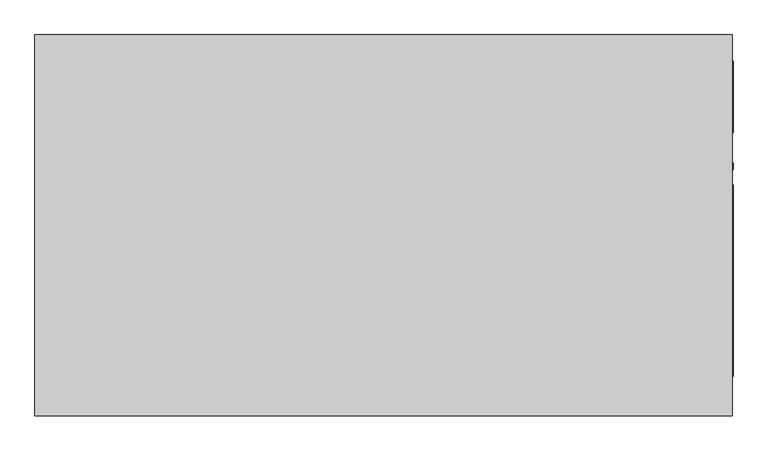
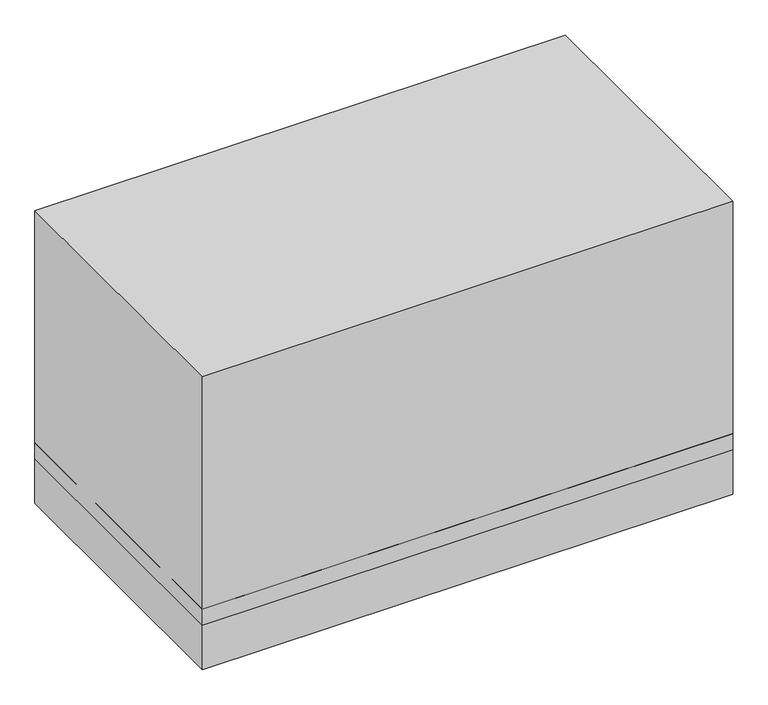
"""IFC4 building model written with IfcOpenShell, lengths in millimetres: proxy geometry, Carrier_48TC_Standard_Efficiency_Gas_Heat_Electric_Cooling_Packaged_Rooftop_Unit_3_to_15_nominal_tons : 15 ton 48TC**16."""

from ifc_helpers import new_model, si_unit, point, frame, frame_2d, origin, origin_with_axes, place, context, project, spatial, polyline, circle_curve, trimmed, segment, composite_curve, outline, extrude, source, transform, mapped, element, save
from ifc_brep_helpers import plane_surface, revolved_surface, advanced_brep


def mechanical_equipment_2a90b6eb(model_context):
    return source(origin(), model_context, "Body", "SolidModel", [
        extrude(outline(composite_curve([segment(trimmed(circle_curve(frame_2d((249.2375, 434.975)), 13.2953125), [point((235.9421875, 434.975))], [point((262.5328125, 434.975))], False, "CARTESIAN"), True, "CONTINUOUS"), segment(trimmed(circle_curve(frame_2d((249.2375, 434.975)), 13.2953125), [point((262.5328125, 434.975))], [point((235.9421875, 434.975))], False, "CARTESIAN"), True, "CONTINUOUS")], self_intersect=False)), frame((1471.6125, 0.0, 0.0), z_axis=(1.0, 0.0, 0.0), x_axis=(0.0, 1.0, 0.0)), (0.0, 0.0, 1.0), 3.175),
        advanced_brep(
        [(1471.6125, 804.8625, 1717.675), (-1471.6125, 804.8625, 1717.675), (-1471.6125, -804.8625, 1717.675), (1471.6125, -804.8625, 1717.675), (1471.6125, 804.8625, 260.35), (1471.6125, -804.8625, 260.35), (-1471.6125, -804.8625, 260.35), (-1471.6125, 804.8625, 260.35), (1312.8625, -681.0375, 260.35), (1312.8625, 0.0, 260.35), (633.4125, 0.0, 260.35), (633.4125, -681.0375, 260.35), (1312.8625, 642.9375, 260.35), (122.2375, 642.9375, 260.35), (122.2375, 322.2625, 260.35), (1312.8625, 322.2625, 260.35), (430.8078125, -144.4625, 260.35), (404.2171875, -144.4625, 260.35), (-336.55, -423.8625, 260.35), (-358.775, -423.8625, 260.35), (-315.9125, -344.4875, 260.35), (-379.4125, -344.4875, 260.35), (-325.4375, -233.3625, 260.35), (-369.8875, -233.3625, 260.35), (1312.8625, -681.0375, 381.0), (633.4125, -681.0375, 381.0), (633.4125, 0.0, 381.0), (1312.8625, 0.0, 381.0), (1312.8625, 642.9375, 381.0), (1312.8625, 322.2625, 381.0), (122.2375, 322.2625, 381.0), (122.2375, 642.9375, 381.0), (430.8078125, -144.4625, 415.925), (404.2171875, -144.4625, 415.925), (-336.55, -423.8625, 415.925), (-358.775, -423.8625, 415.925), (-315.9125, -344.4875, 415.925), (-379.4125, -344.4875, 415.925), (-325.4375, -233.3625, 415.925), (-369.8875, -233.3625, 415.925)],
        [
            (0, 1),
            (1, 2),
            (2, 3),
            (3, 0),
            (4, 5),
            (5, 6),
            (6, 7),
            (7, 4),
            (8, 9),
            (9, 10),
            (10, 11),
            (11, 8),
            (12, 13),
            (13, 14),
            (14, 15),
            (15, 12),
            (16, 17, circle_curve(frame((417.5125, -144.4625, 260.35), z_axis=(0.0, 0.0, 1.0), x_axis=(-1.0, 0.0, 0.0)), 13.2953125)),
            (17, 16, circle_curve(frame((417.5125, -144.4625, 260.35), z_axis=(0.0, 0.0, 1.0), x_axis=(-1.0, 0.0, 0.0)), 13.2953125)),
            (18, 19, circle_curve(frame((-347.6625, -423.8625, 260.35), z_axis=(0.0, 0.0, 1.0), x_axis=(-1.0, 0.0, 0.0)), 11.1125)),
            (19, 18, circle_curve(frame((-347.6625, -423.8625, 260.35), z_axis=(0.0, 0.0, 1.0), x_axis=(-1.0, 0.0, 0.0)), 11.1125)),
            (20, 21, circle_curve(frame((-347.6625, -344.4875, 260.35), z_axis=(0.0, 0.0, 1.0), x_axis=(-1.0, 0.0, 0.0)), 31.75)),
            (21, 20, circle_curve(frame((-347.6625, -344.4875, 260.35), z_axis=(0.0, 0.0, 1.0), x_axis=(-1.0, 0.0, 0.0)), 31.75)),
            (22, 23, circle_curve(frame((-347.6625, -233.3625, 260.35), z_axis=(0.0, 0.0, 1.0), x_axis=(-1.0, 0.0, 0.0)), 22.225)),
            (23, 22, circle_curve(frame((-347.6625, -233.3625, 260.35), z_axis=(0.0, 0.0, 1.0), x_axis=(-1.0, 0.0, 0.0)), 22.225)),
            (0, 4),
            (7, 1),
            (6, 2),
            (5, 3),
            (24, 25),
            (25, 26),
            (26, 27),
            (27, 24),
            (27, 9),
            (8, 24),
            (26, 10),
            (25, 11),
            (28, 29),
            (29, 30),
            (30, 31),
            (31, 28),
            (31, 13),
            (12, 28),
            (30, 14),
            (29, 15),
            (32, 33, circle_curve(frame((417.5125, -144.4625, 415.925), z_axis=(0.0, 0.0, -1.0), x_axis=(-1.0, 0.0, 0.0)), 13.2953125)),
            (33, 32, circle_curve(frame((417.5125, -144.4625, 415.925), z_axis=(0.0, 0.0, -1.0), x_axis=(-1.0, 0.0, 0.0)), 13.2953125)),
            (33, 17),
            (16, 32),
            (34, 35, circle_curve(frame((-347.6625, -423.8625, 415.925), z_axis=(0.0, 0.0, -1.0), x_axis=(-1.0, 0.0, 0.0)), 11.1125)),
            (35, 34, circle_curve(frame((-347.6625, -423.8625, 415.925), z_axis=(0.0, 0.0, -1.0), x_axis=(-1.0, 0.0, 0.0)), 11.1125)),
            (35, 19),
            (18, 34),
            (36, 37, circle_curve(frame((-347.6625, -344.4875, 415.925), z_axis=(0.0, 0.0, -1.0), x_axis=(-1.0, 0.0, 0.0)), 31.75)),
            (37, 36, circle_curve(frame((-347.6625, -344.4875, 415.925), z_axis=(0.0, 0.0, -1.0), x_axis=(-1.0, 0.0, 0.0)), 31.75)),
            (37, 21),
            (20, 36),
            (38, 39, circle_curve(frame((-347.6625, -233.3625, 415.925), z_axis=(0.0, 0.0, -1.0), x_axis=(-1.0, 0.0, 0.0)), 22.225)),
            (39, 38, circle_curve(frame((-347.6625, -233.3625, 415.925), z_axis=(0.0, 0.0, -1.0), x_axis=(-1.0, 0.0, 0.0)), 22.225)),
            (39, 23),
            (22, 38),
        ],
        [
            plane_surface(frame((-1471.6125, 804.8625, 1717.675), z_axis=(0.0, 0.0, 1.0), x_axis=(-1.0, 0.0, 0.0))),
            plane_surface(frame((-1471.6125, 804.8625, 260.35), z_axis=(0.0, 0.0, -1.0), x_axis=(1.0, 0.0, 0.0))),
            plane_surface(frame((1471.6125, 804.8625, 1717.675), z_axis=(0.0, 1.0, 0.0), x_axis=(0.0, 0.0, -1.0))),
            plane_surface(frame((-1471.6125, 804.8625, 1717.675), z_axis=(-1.0, 0.0, 0.0), x_axis=(0.0, 0.0, -1.0))),
            plane_surface(frame((-1471.6125, -804.8625, 1717.675), z_axis=(0.0, -1.0, 0.0), x_axis=(0.0, 0.0, -1.0))),
            plane_surface(frame((1471.6125, -804.8625, 1717.675), z_axis=(1.0, 0.0, 0.0), x_axis=(0.0, 0.0, -1.0))),
            plane_surface(frame((1312.8625, -681.0375, 381.0), z_axis=(0.0, 0.0, -1.0), x_axis=(0.0, 1.0, 0.0))),
            plane_surface(frame((1312.8625, -681.0375, 381.0), z_axis=(-1.0, 0.0, 0.0), x_axis=(0.0, 0.0, -1.0))),
            plane_surface(frame((1312.8625, 0.0, 381.0), z_axis=(0.0, -1.0, 0.0), x_axis=(0.0, 0.0, -1.0))),
            plane_surface(frame((633.4125, 0.0, 381.0), z_axis=(1.0, 0.0, 0.0), x_axis=(0.0, 0.0, -1.0))),
            plane_surface(frame((633.4125, -681.0375, 381.0), z_axis=(0.0, 1.0, 0.0), x_axis=(0.0, 0.0, -1.0))),
            plane_surface(frame((122.2375, 642.9375, 381.0), z_axis=(0.0, 0.0, -1.0), x_axis=(-1.0, 0.0, 0.0))),
            plane_surface(frame((1312.8625, 642.9375, 381.0), z_axis=(0.0, -1.0, 0.0), x_axis=(0.0, 0.0, -1.0))),
            plane_surface(frame((122.2375, 642.9375, 381.0), z_axis=(1.0, 0.0, 0.0), x_axis=(0.0, 0.0, -1.0))),
            plane_surface(frame((122.2375, 322.2625, 381.0), z_axis=(0.0, 1.0, 0.0), x_axis=(0.0, 0.0, -1.0))),
            plane_surface(frame((1312.8625, 322.2625, 381.0), z_axis=(-1.0, 0.0, 0.0), x_axis=(0.0, 0.0, -1.0))),
            plane_surface(frame((404.2171875, -144.4625, 415.925), z_axis=(0.0, 0.0, -1.0), x_axis=(0.0, -1.0, 0.0))),
            revolved_surface(polyline([(404.21718749999997, -144.4625, 415.925), (404.21718749999997, -144.4625, 260.35)]), (417.5125, -144.4625, 0.0), (0.0, 0.0, 1.0)),
            plane_surface(frame((-358.775, -423.8625, 415.925), z_axis=(0.0, 0.0, -1.0), x_axis=(0.0, -1.0, 0.0))),
            revolved_surface(polyline([(-358.77500000000003, -423.8625, 415.925), (-358.77500000000003, -423.8625, 260.35)]), (-347.6625, -423.8625, 0.0), (0.0, 0.0, 1.0)),
            plane_surface(frame((-379.4125, -344.4875, 415.925), z_axis=(0.0, 0.0, -1.0), x_axis=(0.0, -1.0, 0.0))),
            revolved_surface(polyline([(-379.4125, -344.4875, 415.925), (-379.4125, -344.4875, 260.35)]), (-347.6625, -344.4875, 0.0), (0.0, 0.0, 1.0)),
            plane_surface(frame((-369.8875, -233.3625, 415.925), z_axis=(0.0, 0.0, -1.0), x_axis=(0.0, -1.0, 0.0))),
            revolved_surface(polyline([(-369.88750000000005, -233.3625, 415.925), (-369.88750000000005, -233.3625, 260.35)]), (-347.6625, -233.3625, 0.0), (0.0, 0.0, 1.0)),
        ],
        [
            (0, [[1, 2, 3, 4]]),
            (1, [[5, 6, 7, 8], [9, 10, 11, 12], [13, 14, 15, 16], [17, 18], [19, 20], [21, 22], [23, 24]]),
            (2, [[-1, 25, -8, 26]]),
            (3, [[-2, -26, -7, 27]]),
            (4, [[-3, -27, -6, 28]]),
            (5, [[-4, -28, -5, -25]]),
            (6, [[29, 30, 31, 32]]),
            (7, [[-32, 33, -9, 34]]),
            (8, [[-31, 35, -10, -33]]),
            (9, [[-30, 36, -11, -35]]),
            (10, [[-29, -34, -12, -36]]),
            (11, [[37, 38, 39, 40]]),
            (12, [[-40, 41, -13, 42]]),
            (13, [[-39, 43, -14, -41]]),
            (14, [[-38, 44, -15, -43]]),
            (15, [[-37, -42, -16, -44]]),
            (16, [[45, 46]]),
            (17, [[-46, 47, -17, 48]]),
            (17, [[-45, -48, -18, -47]]),
            (18, [[49, 50]]),
            (19, [[-50, 51, -19, 52]]),
            (19, [[-49, -52, -20, -51]]),
            (20, [[53, 54]]),
            (21, [[-54, 55, -21, 56]]),
            (21, [[-53, -56, -22, -55]]),
            (22, [[57, 58]]),
            (23, [[-58, 59, -23, 60]]),
            (23, [[-57, -60, -24, -59]]),
        ],
    ),
        extrude(outline(polyline([(1471.6125, 804.8625), (1471.6125, -804.8625), (-1471.6125, -804.8625), (-1471.6125, 804.8625), (1471.6125, 804.8625)]), holes=[polyline([(1312.8625, 642.9375), (122.2375, 642.9375), (122.2375, 322.2625), (1312.8625, 322.2625), (1312.8625, 642.9375)]), polyline([(1312.8625, -681.0375), (1312.8625, 0.0), (633.4125, 0.0), (633.4125, -681.0375), (1312.8625, -681.0375)]), composite_curve([segment(trimmed(circle_curve(frame_2d((417.5125, -144.4625)), 13.2953125), [point((430.8078125, -144.4625))], [point((404.2171875, -144.4625))], True, "CARTESIAN"), True, "CONTINUOUS"), segment(trimmed(circle_curve(frame_2d((417.5125, -144.4625)), 13.2953125), [point((404.2171875, -144.4625))], [point((430.8078125, -144.4625))], True, "CARTESIAN"), True, "CONTINUOUS")], self_intersect=False), composite_curve([segment(trimmed(circle_curve(frame_2d((-347.6625, -423.8625)), 11.1125), [point((-336.55, -423.8625))], [point((-358.775, -423.8625))], True, "CARTESIAN"), True, "CONTINUOUS"), segment(trimmed(circle_curve(frame_2d((-347.6625, -423.8625)), 11.1125), [point((-358.775, -423.8625))], [point((-336.55, -423.8625))], True, "CARTESIAN"), True, "CONTINUOUS")], self_intersect=False), composite_curve([segment(trimmed(circle_curve(frame_2d((-347.6625, -344.4875)), 31.75), [point((-315.9125, -344.4875))], [point((-379.4125, -344.4875))], True, "CARTESIAN"), True, "CONTINUOUS"), segment(trimmed(circle_curve(frame_2d((-347.6625, -344.4875)), 31.75), [point((-379.4125, -344.4875))], [point((-315.9125, -344.4875))], True, "CARTESIAN"), True, "CONTINUOUS")], self_intersect=False), composite_curve([segment(trimmed(circle_curve(frame_2d((-347.6625, -233.3625)), 22.225), [point((-325.4375, -233.3625))], [point((-369.8875, -233.3625))], True, "CARTESIAN"), True, "CONTINUOUS"), segment(trimmed(circle_curve(frame_2d((-347.6625, -233.3625)), 22.225), [point((-369.8875, -233.3625))], [point((-325.4375, -233.3625))], True, "CARTESIAN"), True, "CONTINUOUS")], self_intersect=False)]), origin_with_axes(), (0.0, 0.0, 1.0), 355.6),
        extrude(outline(polyline([(1474.7875, 693.7375), (1474.7875, 392.1125), (1471.6125, 392.1125), (1471.6125, 693.7375), (1474.7875, 693.7375)])), frame((0.0, 0.0, 415.925), z_axis=(0.0, 0.0, 1.0), x_axis=(1.0, 0.0, 0.0)), (0.0, 0.0, 1.0), 1171.575),
        extrude(outline(polyline([(1474.7875, 169.8625), (1474.7875, -636.5875), (1471.6125, -636.5875), (1471.6125, 169.8625), (1474.7875, 169.8625)])), frame((0.0, 0.0, 415.925), z_axis=(0.0, 0.0, 1.0), x_axis=(1.0, 0.0, 0.0)), (0.0, 0.0, 1.0), 371.475),
    ])


if __name__ == "__main__":
    model = new_model("IFC4")
    model_context = context("Model", 3, world=origin())
    ifc_project = project(units=[si_unit("LENGTHUNIT", "METRE", prefix="MILLI")], contexts=[model_context])
    site = spatial("IfcSite", under=ifc_project)
    building = spatial("IfcBuilding", under=site)
    placement = place(None, origin())
    mechanical_equipment_shape = mechanical_equipment_2a90b6eb(model_context)
    element("IfcBuildingElementProxy", 1, Name="Carrier_48TC_Standard_Efficiency_Gas_Heat_Electric_Cooling_Packaged_Rooftop_Unit_3_to_15_nominal_tons : 15 ton 48TC**16", ObjectType="Carrier_48TC_Standard_Efficiency_Gas_Heat_Electric_Cooling_Packaged_Rooftop_Unit_3_to_15_nominal_tons : 15 ton 48TC**16", at=placement, inside=building, context=model_context, shape_type="MappedRepresentation", body=[
        mapped(mechanical_equipment_shape, transform((0.0, 0.0, 0.0), x_axis=(1.0, 0.0, 0.0), y_axis=(0.0, 1.0, 0.0), z_axis=(0.0, 0.0, 1.0))),
    ])
    save(model, "model.ifc")

# Revit data of these elements
# Type "Carrier_48TC_Standard_Efficiency_Gas_Heat_Electric_Cooling_Packaged_Rooftop_Unit_3_to_15_nominal_tons : 15 ton 48TC**16"
#   URL = "www.Carrier.com"
#   Model = "48TC"
#   Manufacturer = "Carrier"
#   Disclaimer = "Manufacturer reserves the right to change, at any time, specifications and designs without notice and without obligation.  Please verify critical parameters with local Carrier commercial sales office."
#   knockout thickness = 0' - 0 1/16"
#   Voltage = 0 V
#   Version = 1
#   TTBY3 = 1' - 3"
#   TTBY2 = 1' - 6 1/8"
#   TTBY1 = 1' - 10 1/2"
#   TTBX = 3' - 8 1/4"
#   TTBPowerR = 0' - 1 1/4"
#   TTBGasR = 0' - 0 7/8"
#   SSSZ = 0' - 6 1/8"
#   SSSY = 0' - 6 5/8"
#   SSSW = 2' - 7 3/4"
#   SSSH = 1' - 2 5/8"
#   SSRZ = 0' - 6 1/8"
#   SSRY = 0' - 4 3/8"
#   SSRW = 0' - 11 7/8"
#   SSRH = 3' - 10 1/8"
#   SEER = 0
#   Right clearance = 3' - 0"
#   PWRZ = 2' - 11 3/4"
#   PWRY = 0' - 11.71105"
#   PWRR = 0' - 1 1/4"
#   ODF2X = 2' - 1"
#   ODF1Y = 1' - 0"
#   ODF1X = 1' - 1"
#   ODF1R = 0' - 11"
#   MOCP = 0 A
#   MCA = 0 A
#   Left clearance = 4' - 0"
#   IEER = 11.7
#   Front clearance = 4' - 0"
#   Fan Z = 5' - 7 5/8"
#   Width = 5' - 3 3/8"
#   Length = 9' - 7 7/8"
#   Height = 4' - 9 3/8"
#   EER = 10.8
#   DSSY = 0' - 4 7/8"
#   DSSX = 0' - 6 1/4"
#   DSSW = 2' - 2 3/4"
#   DSSH = 2' - 10"
#   DSRY = 0' - 6 3/8"
#   DSRX = 0' - 6 1/4"
#   DSRW = 3' - 10 7/8"
#   DSRH = 1' - 0 5/8"
#   DRNZ = 0' - 6 7/8"
#   DRNY = 3' - 5 1/2"
#   DRNR = 0' - 0 67/128"
#   Curb Z = 1' - 2"
#   CFM (nominal) = 0 CFM
#   Back clearance = 3' - 0"
#   Alt Condensate Drain = 0' - 0 67/128"
#   AccypwrR = 0' - 0 7/16"
#   ACY = 2' - 2"
#   ACX = 3' - 5 1/2"
#   Gas [instance default] = yes
#   Fan 2 on = yes
#   Curb_1SLAB_2ROOFCURB_3SNOWCURB = 2
#   Fan 3 on = yes
#   Unit material = SINGLE-PACKAGED ROOFTOP UNITS
#   Curb material = Curb paint
# Element 1 (IfcBuildingElementProxy, "Carrier_48TC_Standard_Efficiency_Gas_Heat_Electric_Cooling_Packaged_Rooftop_Unit_3_to_15_nominal_tons : 15 ton 48TC**16")
#   Materials on its faces: "SINGLE-PACKAGED ROOFTOP UNITS", "Curb paint", "Mech"
# Materials
#   "SINGLE-PACKAGED ROOFTOP UNITS": class "Miscellaneous", colour RGB 201 201 201, transparency 0, Cost = 0
#   "Curb paint": class "Miscellaneous", colour RGB 189 187 185, transparency 0
#   "Mech": class "Miscellaneous", colour RGB 235 237 235, transparency 0, Cost = 0
